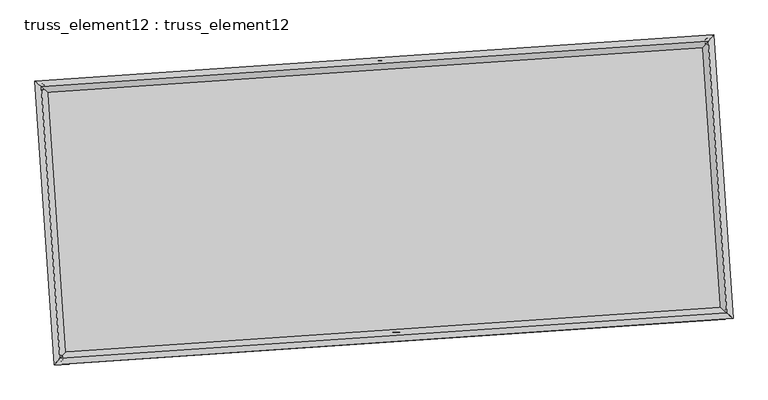
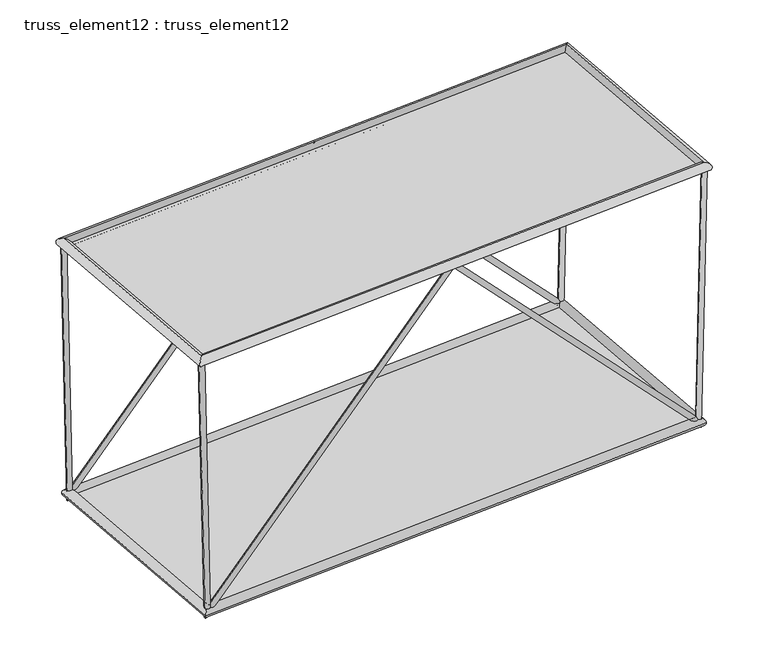
"""IFC4 building model written with IfcOpenShell, lengths in millimetres: plate geometry, truss_element12 : truss_element12."""

from ifc_helpers import new_model, si_unit, frame, origin, origin_with_axes, place, context, project, spatial, polyline, circle_curve, ellipse_curve, outline, extrude, source, transform, mapped, element, save
from ifc_brep_helpers import plane_surface, cylinder_surface, advanced_brep


def truss_element12_truss_element12_d9043aa5(model_context):
    return source(origin(), model_context, "Body", "SolidModel", [
        advanced_brep(
        [(-3779.3847927, 2268.4205144, 4999.8287822), (-3878.4619663, 2255.0610807, 4997.5398535), (-3667.7051723, 2276.0355231, 121.2875859), (-3761.2817105, 2263.0511569, -121.2875859), (1064.0307623, 2598.6746095, 5070.7911995), (1064.4743138, 2592.1011158, 4926.5631841), (5795.1587841, 2921.2722446, 121.2833632), (5889.602193, 2921.1082439, -121.2833632), (5907.4418107, 2928.9283974, 4999.8207113), (6007.4151005, 2929.1414582, 4997.5194202)],
        [
            (0, 1, circle_curve(frame((-3828.9233795, 2261.7407976, 4998.6843179), z_axis=(-0.022885987621300542, -0.0015605084981128968, 0.9997368635715225), x_axis=(-0.1335949015683581, 0.9910348723202073, -0.0015113306095192321)), 50.0)),
            (1, 0, circle_curve(frame((-3828.9233795, 2261.7407976, 4998.6843179), z_axis=(-0.022885987621300542, -0.0015605084981128968, 0.9997368635715225), x_axis=(-0.1335949015683581, 0.9910348723202073, -0.0015113306095192321)), 50.0)),
            (0, 2),
            (2, 3, ellipse_curve(frame((-3714.4934414, 2269.54334, 0.0), z_axis=(-0.9299643254301769, -0.06341073222572768, 0.3621400729908157), x_axis=(0.36130113787628076, 0.024635751157578885, 0.9321236868217687)), 130.4029578, 50.0)),
            (3, 1),
            (3, 2, ellipse_curve(frame((-3714.4934414, 2269.54334, 0.0), z_axis=(-0.9299643254301769, -0.06341073222572768, 0.3621400729908157), x_axis=(0.36130113787628076, 0.024635751157578885, 0.9321236868217687)), 130.4029578, 50.0)),
            (2, 4),
            (4, 5, ellipse_curve(frame((1064.252538, 2595.3878627, 4998.6771918), z_axis=(-0.9976833955542866, -0.06802823819320543, 3.230475386038004e-05), x_axis=(-3.222991654096142e-05, -2.1976354914675906e-06, -0.9999999994782015)), 72.2710337, 50.0)),
            (5, 3),
            (5, 4, ellipse_curve(frame((1064.252538, 2595.3878627, 4998.6771918), z_axis=(-0.9976833955542866, -0.06802823819320543, 3.230475386038004e-05), x_axis=(-3.222991654096142e-05, -2.1976354914675906e-06, -0.9999999994782015)), 72.2710337, 50.0)),
            (4, 6),
            (6, 7, ellipse_curve(frame((5842.3804885, 2921.1902443, 0.0), z_axis=(-0.9299983802713416, -0.06341305429589221, -0.3620522023652769), x_axis=(-0.36121347081217786, -0.024629773473731513, 0.9321578207376972)), 130.3936428, 50.0)),
            (7, 5),
            (7, 6, ellipse_curve(frame((5842.3804885, 2921.1902443, 0.0), z_axis=(-0.9299983802713416, -0.06341305429589221, -0.3620522023652769), x_axis=(-0.36121347081217786, -0.024629773473731513, 0.9321578207376972)), 130.3936428, 50.0)),
            (8, 9, circle_curve(frame((5957.4284556, 2929.0349278, 4998.6700657), z_axis=(0.0230095934179778, 0.0015689367075186376, 0.9997340131496715), x_axis=(-0.002166147289386425, 0.9999964994670225, -0.001519493212205327)), 50.0)),
            (9, 8, circle_curve(frame((5957.4284556, 2929.0349278, 4998.6700657), z_axis=(0.0230095934179778, 0.0015689367075186376, 0.9997340131496715), x_axis=(-0.002166147289386425, 0.9999964994670225, -0.001519493212205327)), 50.0)),
            (6, 8),
            (9, 7),
        ],
        [
            plane_surface(frame((-3828.9233795, 2311.7407366, 4998.7623637), z_axis=(-0.022885987621301448, -0.0015605084981140727, 0.9997368635715226), x_axis=(0.9997380814846446, -3.572313472144376e-05, 0.02288595974085441))),
            cylinder_surface(frame((-3828.9233795, 2261.7407976, 4998.6843179), z_axis=(-0.022885987621300546, -0.0015605084981128972, 0.9997368635715227), x_axis=(-0.1335949015683581, 0.9910348723202073, -0.0015113306095192321)), 50.0),
            cylinder_surface(frame((-3714.4934414, 2269.54334, 0.0), z_axis=(-0.6902606627361213, -0.04706625066554751, -0.7220283827713277), x_axis=(-0.020420229147649776, 0.998751823015369, -0.045583004124724665)), 50.0),
            cylinder_surface(frame((1064.252538, 2595.3878627, 4998.6771918), z_axis=(-0.6902141194664037, -0.04706307705691311, 0.7220730822203193), x_axis=(-0.11534357052060634, 0.9922793612045488, -0.045579930529241086)), 50.0),
            plane_surface(frame((5957.4284556, 2879.0349894, 4998.7485334), z_axis=(0.023009593417979597, 0.0015689367075153572, 0.9997340131496715), x_axis=(0.9997352442575682, -3.611015610971435e-05, -0.023009565083185635))),
            cylinder_surface(frame((5842.3804885, 2921.1902443, 0.0), z_axis=(-0.023009593417977797, -0.0015689367075186372, -0.9997340131496713), x_axis=(-0.002166147289386425, 0.9999964994670225, -0.001519493212205327)), 50.0),
        ],
        [
            (0, [[1, 2]]),
            (1, [[-1, 3, 4, 5]]),
            (1, [[-2, -5, 6, -3]]),
            (2, [[-4, 7, 8, 9]]),
            (2, [[-6, -9, 10, -7]]),
            (3, [[-8, 11, 12, 13]]),
            (3, [[-10, -13, 14, -11]]),
            (4, [[15, 16]]),
            (5, [[-12, 17, -16, 18]]),
            (5, [[-14, -18, -15, -17]]),
        ],
    ),
        advanced_brep(
        [(-3507.2718398, -1722.3130699, 4999.8287822), (-3606.3490134, -1735.6725036, 4997.5398535), (-3395.5922194, -1714.6980612, 121.2875859), (-3489.1687576, -1727.6824274, -121.2875859), (1336.1437152, -1392.0589748, 5070.7911995), (1336.5872667, -1398.6324685, 4926.5631841), (6067.271737, -1069.4613397, 121.2833632), (6161.7151459, -1069.6253404, -121.2833632), (6179.5547636, -1061.8051869, 4999.8207113), (6279.5280534, -1061.5921261, 4997.5194202)],
        [
            (0, 1, circle_curve(frame((-3556.8104266, -1728.9927867, 4998.6843179), z_axis=(-0.022885987621300105, -0.0015605084981129068, 0.9997368635715226), x_axis=(-0.13359490156835802, 0.9910348723202074, -0.001511330609519162)), 50.0)),
            (1, 0, circle_curve(frame((-3556.8104266, -1728.9927867, 4998.6843179), z_axis=(-0.022885987621300105, -0.0015605084981129068, 0.9997368635715226), x_axis=(-0.13359490156835802, 0.9910348723202074, -0.001511330609519162)), 50.0)),
            (0, 2),
            (2, 3, ellipse_curve(frame((-3442.3804885, -1721.1902443, 0.0), z_axis=(-0.9299643254301768, -0.06341073222572771, 0.36214007299081585), x_axis=(0.3613011378762808, 0.024635751157578854, 0.9321236868217686)), 130.4029578, 50.0)),
            (3, 1),
            (3, 2, ellipse_curve(frame((-3442.3804885, -1721.1902443, 0.0), z_axis=(-0.9299643254301768, -0.06341073222572771, 0.36214007299081585), x_axis=(0.3613011378762808, 0.024635751157578854, 0.9321236868217686)), 130.4029578, 50.0)),
            (2, 4),
            (4, 5, ellipse_curve(frame((1336.3654909, -1395.3457216, 4998.6771918), z_axis=(-0.9976833955542866, -0.06802823819320533, 3.230475386021957e-05), x_axis=(-3.222991654080765e-05, -2.19763549153486e-06, -0.9999999994782015)), 72.2710337, 50.0)),
            (5, 3),
            (5, 4, ellipse_curve(frame((1336.3654909, -1395.3457216, 4998.6771918), z_axis=(-0.9976833955542866, -0.06802823819320533, 3.230475386021957e-05), x_axis=(-3.222991654080765e-05, -2.19763549153486e-06, -0.9999999994782015)), 72.2710337, 50.0)),
            (4, 6),
            (6, 7, ellipse_curve(frame((6114.4934414, -1069.54334, 0.0), z_axis=(-0.9299983802713416, -0.06341305429589225, -0.3620522023652771), x_axis=(-0.3612134708121779, -0.02462977347373136, 0.9321578207376972)), 130.3936428, 50.0)),
            (7, 5),
            (7, 6, ellipse_curve(frame((6114.4934414, -1069.54334, 0.0), z_axis=(-0.9299983802713416, -0.06341305429589225, -0.3620522023652771), x_axis=(-0.3612134708121779, -0.02462977347373136, 0.9321578207376972)), 130.3936428, 50.0)),
            (8, 9, circle_curve(frame((6229.5414085, -1061.6986565, 4998.6700657), z_axis=(0.023009593417977526, 0.0015689367075187803, 0.9997340131496715), x_axis=(-0.0021661472893863346, 0.9999964994670225, -0.0015194932122054722)), 50.0)),
            (9, 8, circle_curve(frame((6229.5414085, -1061.6986565, 4998.6700657), z_axis=(0.023009593417977526, 0.0015689367075187803, 0.9997340131496715), x_axis=(-0.0021661472893863346, 0.9999964994670225, -0.0015194932122054722)), 50.0)),
            (6, 8),
            (9, 7),
        ],
        [
            plane_surface(frame((-3556.8104266, -1678.9928477, 4998.7623637), z_axis=(-0.022885987621301448, -0.0015605084981140768, 0.9997368635715226), x_axis=(0.9997380814846446, -3.572313472144376e-05, 0.02288595974085441))),
            cylinder_surface(frame((-3556.8104266, -1728.9927867, 4998.6843179), z_axis=(-0.022885987621300105, -0.0015605084981129068, 0.9997368635715226), x_axis=(-0.13359490156835802, 0.9910348723202074, -0.001511330609519162)), 50.0),
            cylinder_surface(frame((-3442.3804885, -1721.1902443, 0.0), z_axis=(-0.6902606627361211, -0.04706625066554749, -0.722028382771328), x_axis=(-0.020420229147649727, 0.998751823015369, -0.04558300412472467)), 50.0),
            cylinder_surface(frame((1336.3654909, -1395.3457216, 4998.6771918), z_axis=(-0.6902141194664038, -0.04706307705691299, 0.7220730822203194), x_axis=(-0.11534357052060609, 0.992279361204549, -0.04557993052924103)), 50.0),
            plane_surface(frame((6229.5414085, -1111.6985949, 4998.7485334), z_axis=(0.023009593417976044, 0.0015689367075153572, 0.9997340131496715), x_axis=(0.9997352442575682, -3.611015610971435e-05, -0.023009565083182082))),
            cylinder_surface(frame((6114.4934414, -1069.54334, 0.0), z_axis=(-0.023009593417977522, -0.0015689367075187798, -0.9997340131496713), x_axis=(-0.0021661472893863346, 0.9999964994670225, -0.0015194932122054722)), 50.0),
        ],
        [
            (0, [[1, 2]]),
            (1, [[-1, 3, 4, 5]]),
            (1, [[-2, -5, 6, -3]]),
            (2, [[-4, 7, 8, 9]]),
            (2, [[-6, -9, 10, -7]]),
            (3, [[-8, 11, 12, 13]]),
            (3, [[-10, -13, 14, -11]]),
            (4, [[15, 16]]),
            (5, [[-12, 17, -16, 18]]),
            (5, [[-14, -18, -15, -17]]),
        ],
    ),
        advanced_brep(
        [(-3556.8141269, -1728.996888, 4908.6843179), (-3556.8067263, -1728.9886855, 5088.6843178), (-3828.9191567, 2261.7372366, 5088.6843178), (-3828.9276023, 2261.7443585, 4908.6843179), (5957.4250162, 2929.0308444, 5088.6700657), (5957.431895, 2929.0390112, 4908.6700658), (6229.5374466, -1061.6950777, 5088.6700657), (6229.5453704, -1061.7022353, 4908.6700658)],
        [
            (0, 1, ellipse_curve(frame((-3556.8104266, -1728.9927867, 4998.6843179), z_axis=(-0.7535719234047111, 0.6573654662781341, 1.0273917260532269e-06), x_axis=(-0.6573654662773387, -0.7535719234054049, 1.0273917260533834e-06)), 127.2792206, 90.0)),
            (1, 2),
            (2, 3, ellipse_curve(frame((-3828.9233795, 2261.7407976, 4998.6843179), z_axis=(-0.6573654662773385, -0.7535719234054051, 1.0273917260535286e-06), x_axis=(0.7535719234047112, -0.6573654662781339, -1.0273917260533723e-06)), 127.2792206, 90.0)),
            (3, 0),
            (1, 0, ellipse_curve(frame((-3556.8104266, -1728.9927867, 4998.6843179), z_axis=(-0.7535719234047111, 0.6573654662781341, 1.0273917260532269e-06), x_axis=(-0.6573654662773387, -0.7535719234054049, 1.0273917260533834e-06)), 127.2792206, 90.0)),
            (3, 2, ellipse_curve(frame((-3828.9233795, 2261.7407976, 4998.6843179), z_axis=(-0.6573654662773385, -0.7535719234054051, 1.0273917260535286e-06), x_axis=(0.7535719234047112, -0.6573654662781339, -1.0273917260533723e-06)), 127.2792206, 90.0)),
            (2, 4),
            (4, 5, ellipse_curve(frame((5957.4284556, 2929.0349278, 4998.6700657), z_axis=(-0.7535719234047108, 0.6573654662781345, 1.027391726053518e-06), x_axis=(-0.6573654662773392, -0.7535719234054046, 1.0273917260533831e-06)), 127.2792206, 90.0)),
            (5, 3),
            (5, 4, ellipse_curve(frame((5957.4284556, 2929.0349278, 4998.6700657), z_axis=(-0.7535719234047108, 0.6573654662781345, 1.027391726053518e-06), x_axis=(-0.6573654662773392, -0.7535719234054046, 1.0273917260533831e-06)), 127.2792206, 90.0)),
            (4, 6),
            (6, 7, ellipse_curve(frame((6229.5414085, -1061.6986565, 4998.6700657), z_axis=(0.657365466277339, 0.7535719234054045, -1.0273917260532377e-06), x_axis=(-0.7535719234047105, 0.6573654662781346, 1.0273917260533721e-06)), 127.2792206, 90.0)),
            (7, 5),
            (7, 6, ellipse_curve(frame((6229.5414085, -1061.6986565, 4998.6700657), z_axis=(0.657365466277339, 0.7535719234054045, -1.0273917260532377e-06), x_axis=(-0.7535719234047105, 0.6573654662781346, 1.0273917260533721e-06)), 127.2792206, 90.0)),
            (6, 1),
            (0, 7),
        ],
        [
            cylinder_surface(frame((-3556.8104266, -1728.9927867, 4998.6843179), z_axis=(0.06802823822869865, -0.9976833960748769, 0.0), x_axis=(-0.9976833951038622, -0.06802823816248885, 4.411959662306044e-05)), 90.0),
            cylinder_surface(frame((-3828.9233795, 2261.7407976, 4998.6843179), z_axis=(-0.9976833960738238, -0.06802823822862583, 1.4529513128546934e-06), x_axis=(-0.06802823810492795, 0.9976833951709815, 4.266664531152834e-05)), 90.0),
            cylinder_surface(frame((5957.4284556, 2929.0349278, 4998.6700657), z_axis=(-0.06802823822869723, 0.9976833960748768, 0.0), x_axis=(0.99768339522756, 0.06802823817092192, 4.121369399999627e-05)), 90.0),
            cylinder_surface(frame((6229.5414085, -1061.6986565, 4998.6700657), z_axis=(0.9976833960738238, 0.0680282382286254, -1.452951312854488e-06), x_axis=(0.0680282382286254, -0.997683395162547, 4.2666645311528356e-05)), 90.0),
        ],
        [
            (0, [[1, 2, 3, 4]]),
            (0, [[5, -4, 6, -2]]),
            (1, [[-3, 7, 8, 9]]),
            (1, [[-6, -9, 10, -7]]),
            (2, [[-8, 11, 12, 13]]),
            (2, [[-10, -13, 14, -11]]),
            (3, [[-12, 15, -1, 16]]),
            (3, [[-14, -16, -5, -15]]),
        ],
    ),
        advanced_brep(
        [(-3358.7115243, -1625.2761972, 0.0), (-3526.0494527, -1817.1042913, 0.0), (-3810.4074885, 2353.2123043, 0.0), (-3618.5793943, 2185.8743758, 0.0), (5926.0494527, 3017.1042913, 0.0), (5758.7115243, 2825.2761972, 0.0), (6210.4074885, -1153.2123043, 0.0), (6018.5793943, -985.8743758, 0.0)],
        [
            (0, 1, ellipse_curve(frame((-3442.3804885, -1721.1902443, 0.0), z_axis=(-0.7535719234054589, 0.6573654662780799, 0.0), x_axis=(-0.65736546627808, -0.7535719234054586, 0.0)), 127.2792206, 90.0)),
            (1, 2),
            (2, 3, ellipse_curve(frame((-3714.4934414, 2269.54334, 0.0), z_axis=(-0.6573654662780799, -0.7535719234054586, 0.0), x_axis=(0.7535719234054586, -0.6573654662780801, 0.0)), 127.2792206, 90.0)),
            (3, 0),
            (1, 0, ellipse_curve(frame((-3442.3804885, -1721.1902443, 0.0), z_axis=(-0.7535719234054589, 0.6573654662780799, 0.0), x_axis=(-0.65736546627808, -0.7535719234054586, 0.0)), 127.2792206, 90.0)),
            (3, 2, ellipse_curve(frame((-3714.4934414, 2269.54334, 0.0), z_axis=(-0.6573654662780799, -0.7535719234054586, 0.0), x_axis=(0.7535719234054586, -0.6573654662780801, 0.0)), 127.2792206, 90.0)),
            (2, 4),
            (4, 5, ellipse_curve(frame((5842.3804885, 2921.1902443, 0.0), z_axis=(-0.7535719234054585, 0.6573654662780801, 0.0), x_axis=(-0.6573654662780801, -0.7535719234054586, 0.0)), 127.2792206, 90.0)),
            (5, 3),
            (5, 4, ellipse_curve(frame((5842.3804885, 2921.1902443, 0.0), z_axis=(-0.7535719234054585, 0.6573654662780801, 0.0), x_axis=(-0.6573654662780801, -0.7535719234054586, 0.0)), 127.2792206, 90.0)),
            (4, 6),
            (6, 7, ellipse_curve(frame((6114.4934414, -1069.54334, 0.0), z_axis=(0.65736546627808, 0.7535719234054584, 0.0), x_axis=(-0.7535719234054583, 0.6573654662780803, 0.0)), 127.2792206, 90.0)),
            (7, 5),
            (7, 6, ellipse_curve(frame((6114.4934414, -1069.54334, 0.0), z_axis=(0.65736546627808, 0.7535719234054584, 0.0), x_axis=(-0.7535719234054583, 0.6573654662780803, 0.0)), 127.2792206, 90.0)),
            (6, 1),
            (0, 7),
        ],
        [
            cylinder_surface(frame((-3442.3804885, -1721.1902443, 0.0), z_axis=(0.0680282382287028, -0.9976833960748764, 0.0), x_axis=(-0.9976833960748764, -0.0680282382287028, 0.0)), 90.0),
            cylinder_surface(frame((-3714.4934414, 2269.54334, 0.0), z_axis=(-0.9976833960748765, -0.06802823822870228, 0.0), x_axis=(-0.06802823822870228, 0.9976833960748765, 0.0)), 90.0),
            cylinder_surface(frame((5842.3804885, 2921.1902443, 0.0), z_axis=(-0.06802823822870217, 0.9976833960748765, 0.0), x_axis=(0.9976833960748765, 0.06802823822870217, 0.0)), 90.0),
            cylinder_surface(frame((6114.4934414, -1069.54334, 0.0), z_axis=(0.9976833960748765, 0.06802823822870213, 0.0), x_axis=(0.06802823822870213, -0.9976833960748765, 0.0)), 90.0),
        ],
        [
            (0, [[1, 2, 3, 4]]),
            (0, [[5, -4, 6, -2]]),
            (1, [[-3, 7, 8, 9]]),
            (1, [[-6, -9, 10, -7]]),
            (2, [[-8, 11, 12, 13]]),
            (2, [[-10, -13, 14, -11]]),
            (3, [[-12, 15, -1, 16]]),
            (3, [[-14, -16, -5, -15]]),
        ],
    ),
        extrude(outline(polyline([(-3442.3804885, -1721.1902443), (-3714.4934414, 2269.54334), (5842.3804885, 2921.1902443), (6114.4934414, -1069.54334), (-3442.3804885, -1721.1902443)])), origin_with_axes(), (0.0, 0.0, 1.0), 20.0),
        extrude(outline(polyline([(-1999.9999999, 4904.5377891), (2000.0000001, 4904.537789), (2000.0, -4904.5377891), (-2000.0, -4904.537789), (-1999.9999999, 4904.5377891)])), frame((1200.3090145, 600.0210705, 4998.6771918), z_axis=(1.4495854001402175e-06, 9.884171804557912e-08, 0.9999999999989445), x_axis=(-0.06802823822870323, 0.9976833960748764, 0.0)), (0.0, 0.0, 1.0), 20.0),
    ])


if __name__ == "__main__":
    model = new_model("IFC4")
    model_context = context("Model", 3, world=origin())
    ifc_project = project(units=[si_unit("LENGTHUNIT", "METRE", prefix="MILLI")], contexts=[model_context])
    site = spatial("IfcSite", under=ifc_project)
    building = spatial("IfcBuilding", under=site)
    placement = place(None, origin())
    truss_element12_truss_element12_shape = truss_element12_truss_element12_d9043aa5(model_context)
    element("IfcPlate", 1, ObjectType="truss_element12 : truss_element12", at=placement, inside=building, context=model_context, shape_type="MappedRepresentation", body=[
        mapped(truss_element12_truss_element12_shape, transform((0.0, 0.0, 0.0), x_axis=(1.0, 0.0, 0.0), y_axis=(0.0, 1.0, 0.0), z_axis=(0.0, 0.0, 1.0))),
    ])
    save(model, "model.ifc")

# Revit data of these elements
# Type "truss_element12 : truss_element12"
#   steellbar1 = 90 mm
#   steelbar2 = 50 mm
#   offset1 = 5000 mm
#   M = Default Roof
# Element 1 (IfcPlate, "truss_element12 : truss_element12")
#   Materials on its faces: "Default Roof"
# Materials
#   "Default Roof": class "Miscellaneous", colour RGB 0 127 0, transparency 0, Comments = "Rendering appearance not upgraded Rendering appearance not upgraded ", Cost = 0
